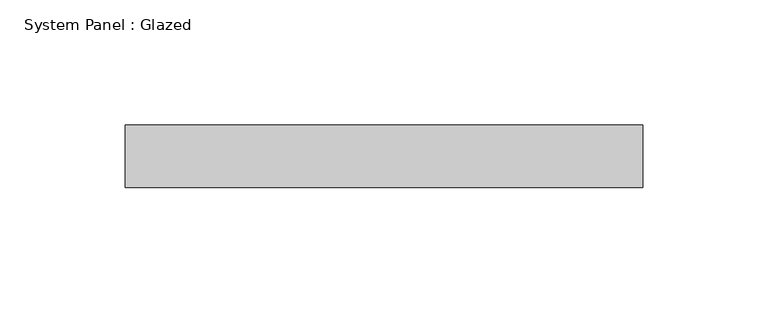
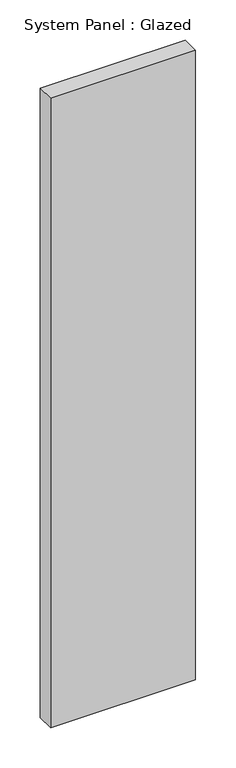
"""IFC4 building model written with IfcOpenShell, lengths in millimetres: plate geometry, System Panel : Glazed."""

from ifc_helpers import new_model, si_unit, origin, origin_with_axes, place, context, project, spatial, polyline, outline, extrude, source, transform, mapped, element, save


def system_panel_glazed_c71140f3(model_context):
    return source(origin(), model_context, "Body", "SweptSolid", [
        extrude(outline(polyline([(103.4090909, 24.5), (-103.4090909, 24.5), (-103.4090909, 49.5), (103.4090909, 49.5), (103.4090909, 24.5)])), origin_with_axes(), (0.0, 0.0, 1.0), 950.0),
    ])


if __name__ == "__main__":
    model = new_model("IFC4")
    model_context = context("Model", 3, world=origin())
    ifc_project = project(units=[si_unit("LENGTHUNIT", "METRE", prefix="MILLI")], contexts=[model_context])
    site = spatial("IfcSite", under=ifc_project)
    building = spatial("IfcBuilding", under=site)
    placement = place(None, origin())
    system_panel_glazed_shape = system_panel_glazed_c71140f3(model_context)
    element("IfcPlate", 1, ObjectType="System Panel : Glazed", at=placement, inside=building, context=model_context, shape_type="MappedRepresentation", body=[
        mapped(system_panel_glazed_shape, transform((0.0, 0.0, 0.0), x_axis=(1.0, 0.0, 0.0), y_axis=(0.0, 1.0, 0.0), z_axis=(0.0, 0.0, 1.0))),
    ])
    save(model, "model.ifc")

# Revit data of these elements
# Element 1 (IfcPlate, "System Panel : Glazed")
#   Materials on its faces: "Glass"
# Materials
#   "Glass": class "Glass", colour RGB 218 227 224, transparency 0.85, Description = "Soda Lime Glass", Cost = 0
